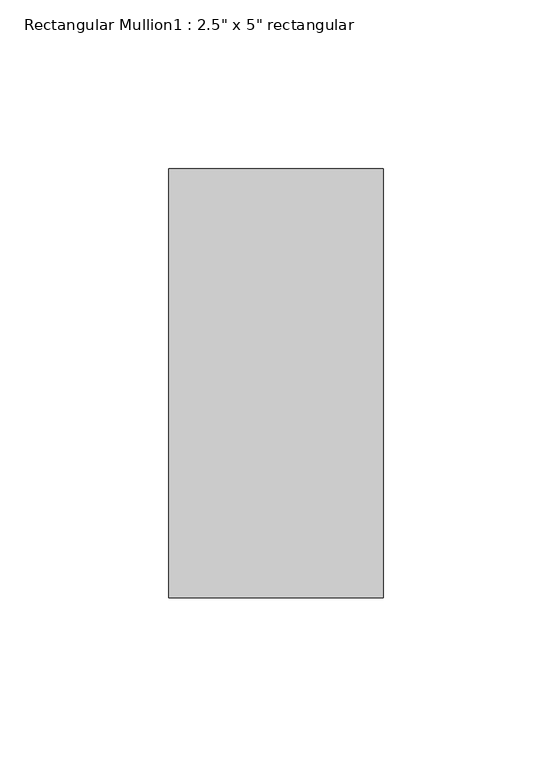
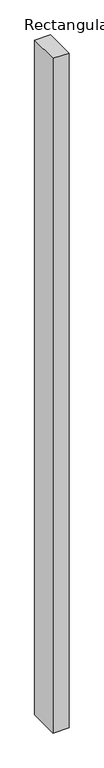
"""IFC4 building model written with IfcOpenShell, lengths in millimetres: member geometry."""

from ifc_helpers import new_model, si_unit, frame, origin, place, context, project, spatial, polyline, outline, extrude, source, transform, mapped, element, save


def member_d1cb1681(model_context):
    return source(origin(), model_context, "Body", "SweptSolid", [
        extrude(outline(polyline([(31.75, 63.5), (31.75, -63.5), (-31.75, -63.5), (-31.75, 63.5), (31.75, 63.5)])), frame((0.0, 0.0, -2852.42), z_axis=(0.0, 0.0, 1.0), x_axis=(1.0, 0.0, 0.0)), (0.0, 0.0, 1.0), 2852.42),
    ])


if __name__ == "__main__":
    model = new_model("IFC4")
    model_context = context("Model", 3, world=origin())
    ifc_project = project(units=[si_unit("LENGTHUNIT", "METRE", prefix="MILLI")], contexts=[model_context])
    site = spatial("IfcSite", under=ifc_project)
    building = spatial("IfcBuilding", under=site)
    placement = place(None, origin())
    member_shape = member_d1cb1681(model_context)
    element("IfcMember", 1, ObjectType="Rectangular Mullion1 : 2.5\" x 5\" rectangular", at=placement, inside=building, context=model_context, shape_type="MappedRepresentation", body=[
        mapped(member_shape, transform((0.0, 0.0, 0.0), x_axis=(1.0, 0.0, 0.0), y_axis=(0.0, 1.0, 0.0), z_axis=(0.0, 0.0, 1.0))),
    ])
    save(model, "model.ifc")

# Revit data of these elements
# Type "Rectangular Mullion1 : 2.5\" x 5\" rectangular"
#   built-in parameter 1007304 = 0.416667 (stored number, unit not read)
#   built-in parameter 1007301 = 0.104167 (stored number, unit not read)
#   built-in parameter 1007300 = 0.104167 (stored number, unit not read)
# Element 1 (IfcMember, "Rectangular Mullion1 : 2.5\" x 5\" rectangular")
#   Materials on its faces: "support-frame"
# Materials
#   "support-frame": class "Unassigned", colour RGB 233 233 233, transparency 0, Cost = 0
